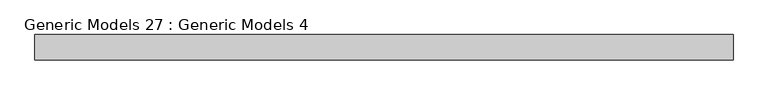
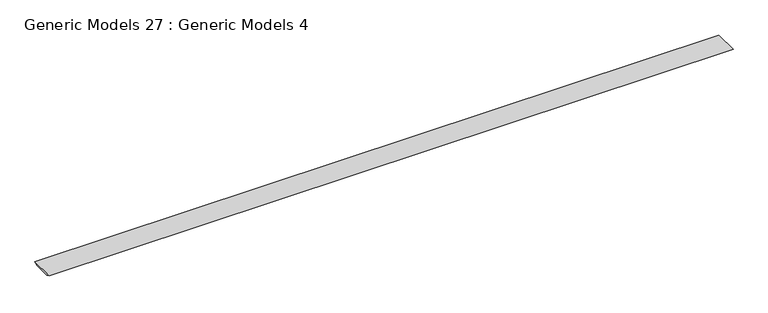
"""IFC4 building model written with IfcOpenShell, lengths in millimetres: proxy geometry, Generic Models 27 : Generic Models 4."""

import ifcopenshell
import ifcopenshell.guid

model = None  # the IFC model being written
_history = None  # IfcOwnerHistory: only IFC2X3 demands one
_inside = {}  # id of a spatial element -> (the spatial element, [elements in it])
_under = {}  # id of a project, library or spatial element -> (it, [spatial elements below it])
_declared = {}  # id of a project -> (the project, [libraries it declares])
_typed = {}  # id of a type object -> (the type object, [elements of that type])
_made_of = {}  # id of a material, layer set ... -> (it, [elements and type objects made of it])


def new_model(schema):
    """Start an empty IFC model of exactly this schema.

    Asked for "IFC4X3", IfcOpenShell would pick the latest addendum, in which some entities
    have other attributes; the version numbers below select the first issue.
    IFC2X3 requires an IfcOwnerHistory on every rooted entity: one is made here for all.
    """
    global model, _history
    if schema == "IFC4X3":
        model = ifcopenshell.file(schema_version=(4, 3, 0, 0))
    else:
        model = ifcopenshell.file(schema=schema)
    _inside.clear()
    _under.clear()
    _declared.clear()
    _typed.clear()
    _made_of.clear()
    _history = None
    if model.schema == "IFC2X3":
        org = make("IfcOrganization", Name="unknown")
        user = make(
            "IfcPersonAndOrganization",
            ThePerson=make("IfcPerson", FamilyName="unknown"),
            TheOrganization=org,
        )
        app = make(
            "IfcApplication",
            ApplicationDeveloper=org,
            Version="unknown",
            ApplicationFullName="unknown",
            ApplicationIdentifier="unknown",
        )
        _history = make(
            "IfcOwnerHistory",
            OwningUser=user,
            OwningApplication=app,
            ChangeAction="ADDED",
            CreationDate=0,
        )
    return model


def make(cls, **values):
    """One entity of the class cls with the attributes given. An attribute that is None is left unset."""
    return model.create_entity(
        cls, **{name: value for name, value in values.items() if value is not None}
    )


def rooted(cls, **values):
    """An entity with a GlobalId (a new one), such as an element, a storey or a relation."""
    return make(cls, GlobalId=ifcopenshell.guid.new(), OwnerHistory=_history, **values)


def si_unit(unit_type, name, prefix=None):
    """IfcSIUnit, for example si_unit("LENGTHUNIT", "METRE", prefix="MILLI")."""
    return make("IfcSIUnit", UnitType=unit_type, Prefix=prefix, Name=name)


def assignment(units):
    """IfcUnitAssignment: the units of a project."""
    return None if units is None else make("IfcUnitAssignment", Units=units)


def point(xyz):
    """IfcCartesianPoint."""
    return None if xyz is None else make("IfcCartesianPoint", Coordinates=xyz)


def direction(xyz):
    """IfcDirection."""
    return None if xyz is None else make("IfcDirection", DirectionRatios=xyz)


def frame(location, z_axis=None, x_axis=None):
    """IfcAxis2Placement3D, a coordinate frame: its origin and axes. An axis left out is left unset."""
    return make(
        "IfcAxis2Placement3D",
        Location=point(location),
        Axis=direction(z_axis),
        RefDirection=direction(x_axis),
    )


def origin():
    """The frame at (0, 0, 0) with its axes left unset."""
    return frame((0.0, 0.0, 0.0))


def place(relative_to, where):
    """IfcLocalPlacement: puts the frame where relative to a parent placement (None: the world)."""
    return make(
        "IfcLocalPlacement", PlacementRelTo=relative_to, RelativePlacement=where
    )


def context(
    kind, dimensions, precision=None, world=None, true_north=None, identifier=None
):
    """IfcGeometricRepresentationContext, for example the 3D "Model" context."""
    return make(
        "IfcGeometricRepresentationContext",
        ContextIdentifier=identifier,
        ContextType=kind,
        CoordinateSpaceDimension=dimensions,
        Precision=precision,
        WorldCoordinateSystem=world,
        TrueNorth=true_north,
    )


def project(units=None, contexts=None):
    """IfcProject with its units and contexts."""
    return rooted(
        "IfcProject",
        Name="project",
        RepresentationContexts=contexts,
        UnitsInContext=assignment(units),
    )


def spatial(cls, under=None, at=None, **own):
    """A site, building, storey or space (cls), placed at a placement, below another one or the project."""
    s = rooted(cls, ObjectPlacement=at, **own)
    if under is not None:
        _under.setdefault(under.id(), (under, []))[1].append(s)
    return s


def polyline(points):
    """IfcPolyline through the points."""
    return make("IfcPolyline", Points=[point(p) for p in points])


def outline(outer, holes=None, kind="AREA"):
    """IfcArbitraryClosedProfileDef: a profile drawn as a closed curve; with holes, ...WithVoids."""
    if holes is None:
        return make("IfcArbitraryClosedProfileDef", ProfileType=kind, OuterCurve=outer)
    return make(
        "IfcArbitraryProfileDefWithVoids",
        ProfileType=kind,
        OuterCurve=outer,
        InnerCurves=holes,
    )


def extrude(swept, where, along, depth):
    """IfcExtrudedAreaSolid: the profile swept, set in the frame where, extruded along a direction by depth."""
    return make(
        "IfcExtrudedAreaSolid",
        SweptArea=swept,
        Position=where,
        ExtrudedDirection=direction(along),
        Depth=depth,
    )


def shape(context_of_items, identifier, shape_type, items):
    """IfcShapeRepresentation: the items that make up one representation, for example the "Body"."""
    return make(
        "IfcShapeRepresentation",
        ContextOfItems=context_of_items,
        RepresentationIdentifier=identifier,
        RepresentationType=shape_type,
        Items=items,
    )


def source(mapping_origin, context_of_items, identifier, shape_type, items):
    """IfcRepresentationMap: a shape defined once, which mapped items show again and again."""
    return make(
        "IfcRepresentationMap",
        MappingOrigin=mapping_origin,
        MappedRepresentation=shape(context_of_items, identifier, shape_type, items),
    )


def transform(
    local_origin,
    x_axis=None,
    y_axis=None,
    z_axis=None,
    scale=None,
    scale2=None,
    scale3=None,
    uniform=True,
):
    """IfcCartesianTransformationOperator3D, or its non-uniform kind. x_axis, y_axis, z_axis: its Axis1, 2, 3."""
    if uniform:
        return make(
            "IfcCartesianTransformationOperator3D",
            Axis1=direction(x_axis),
            Axis2=direction(y_axis),
            LocalOrigin=point(local_origin),
            Scale=scale,
            Axis3=direction(z_axis),
        )
    return make(
        "IfcCartesianTransformationOperator3DnonUniform",
        Axis1=direction(x_axis),
        Axis2=direction(y_axis),
        LocalOrigin=point(local_origin),
        Scale=scale,
        Axis3=direction(z_axis),
        Scale2=scale2,
        Scale3=scale3,
    )


def mapped(mapping_source, mapping_target):
    """IfcMappedItem: shows the shape of a source again, moved by a transform."""
    return make(
        "IfcMappedItem", MappingSource=mapping_source, MappingTarget=mapping_target
    )


def made_of(thing, what):
    """Note that an element or type object is made of a material, layer set ...; save() writes the relation."""
    if what is not None:
        _made_of.setdefault(what.id(), (what, []))[1].append(thing)
    return thing


def element(
    cls,
    number,
    at=None,
    inside=None,
    cuts=None,
    type_object=None,
    material=None,
    context=None,
    identifier="Body",
    shape_type=None,
    held_by="IfcProductDefinitionShape",
    body=None,
    shapes=None,
    **own,
):
    """One element of the class cls, such as IfcWall. Its Tag is "e" and its number.

    at: its placement. inside: the storey or other place that contains it. cuts: it is an
    opening in that element (IfcRelVoidsElement). A single representation is given by context,
    identifier, shape_type and body (its items); several are given by shapes. held_by: the class
    of the entity that holds the representations. save() writes the other relations.
    """
    e = rooted(cls, Tag="e%d" % number, ObjectPlacement=at, **own)
    if body is not None:
        shapes = [shape(context, identifier, shape_type, body)]
    if shapes is not None:
        e.Representation = make(held_by, Representations=shapes)
    if inside is not None:
        _inside.setdefault(inside.id(), (inside, []))[1].append(e)
    if cuts is not None:
        rooted(
            "IfcRelVoidsElement", RelatingBuildingElement=cuts, RelatedOpeningElement=e
        )
    if type_object is not None:
        _typed.setdefault(type_object.id(), (type_object, []))[1].append(e)
    return made_of(e, material)


def aggregate(whole, parts):
    """IfcRelAggregates: a whole, such as a stair, and the parts it consists of."""
    return rooted("IfcRelAggregates", RelatingObject=whole, RelatedObjects=parts)


def save(model, path):
    """Write the relations noted so far, then the file.

    IfcRelAggregates (storeys below a building ...), IfcRelContainedInSpatialStructure (elements
    in a storey), IfcRelDefinesByType, IfcRelAssociatesMaterial and IfcRelDeclares: one each for
    every whole, place, type object, material and project.
    """
    for whole, parts in _under.values():
        aggregate(whole, parts)
    for where, things in _inside.values():
        rooted(
            "IfcRelContainedInSpatialStructure",
            RelatedElements=things,
            RelatingStructure=where,
        )
    for kind, things in _typed.values():
        rooted("IfcRelDefinesByType", RelatedObjects=things, RelatingType=kind)
    for what, things in _made_of.values():
        rooted("IfcRelAssociatesMaterial", RelatedObjects=things, RelatingMaterial=what)
    for by, libraries in _declared.values():
        rooted("IfcRelDeclares", RelatingContext=by, RelatedDefinitions=libraries)
    model.write(path)


def generic_models_27_generic_models_4_9e66ce32(model_context):
    return source(origin(), model_context, "Body", "SweptSolid", [
        extrude(outline(polyline([(-6907.3562447, 127085.8298605), (-7062.7368447, 127089.0145612), (-7098.8080559, 127107.5376156), (-6874.053973, 127102.931027), (-6907.3562447, 127085.8298605)])), frame((2196.9263704, 0.0, 0.0), z_axis=(1.0, 0.0, 0.0), x_axis=(0.0, 1.0, 0.0)), (0.0, 0.0, 1.0), 6212.156498),
    ])


if __name__ == "__main__":
    model = new_model("IFC4")
    model_context = context("Model", 3, world=origin())
    ifc_project = project(units=[si_unit("LENGTHUNIT", "METRE", prefix="MILLI")], contexts=[model_context])
    site = spatial("IfcSite", under=ifc_project)
    building = spatial("IfcBuilding", under=site)
    placement = place(None, origin())
    generic_models_27_generic_models_4_shape = generic_models_27_generic_models_4_9e66ce32(model_context)
    element("IfcBuildingElementProxy", 1, Name="Generic Models 27 : Generic Models 4", ObjectType="Generic Models 27 : Generic Models 4", at=placement, inside=building, context=model_context, shape_type="MappedRepresentation", body=[
        mapped(generic_models_27_generic_models_4_shape, transform((0.0, 0.0, 0.0), x_axis=(1.0, 0.0, 0.0), y_axis=(0.0, 1.0, 0.0), z_axis=(0.0, 0.0, 1.0))),
    ])
    save(model, "model.ifc")

# Revit data of these elements
# Element 1 (IfcBuildingElementProxy, "Generic Models 27 : Generic Models 4")
#   Materials on its faces: "_7/8\" SMOOTH TROWEL EXTERIOR STUCCO (COLOR PER OWNER) @ 2% SLOPE"
# Materials
#   "_7/8\" SMOOTH TROWEL EXTERIOR STUCCO (COLOR PER OWNER) @ 2% SLOPE": class "Generic", colour RGB 233 233 233, transparency 0, Cost = 0
